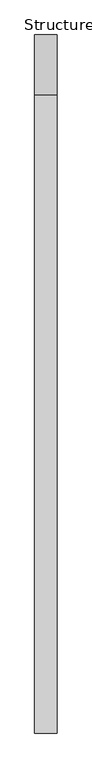
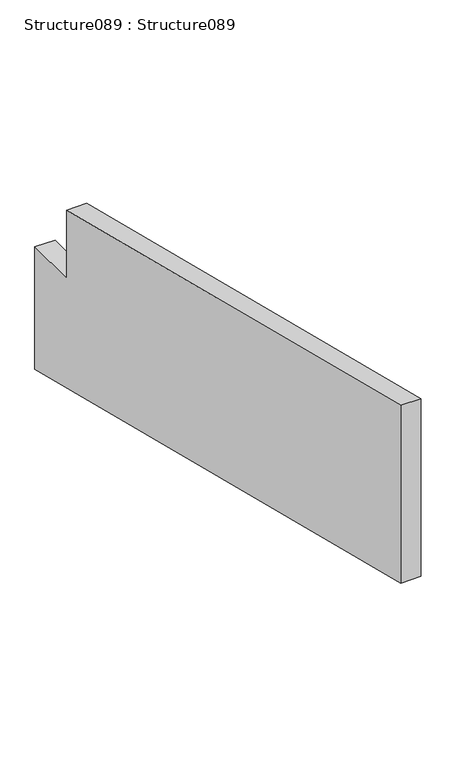
"""IFC4 building model written with IfcOpenShell, lengths in millimetres: proxy geometry, Structure089 : Structure089."""

from ifc_helpers import new_model, si_unit, frame, origin, place, context, project, spatial, polyline, outline, extrude, source, transform, mapped, element, save


def structure089_structure089_4cdf4332(model_context):
    return source(origin(), model_context, "Body", "SweptSolid", [
        extrude(outline(polyline([(3064.1094171, 41796.3564587), (4341.2980909, 41477.0623881), (4341.2980909, 41318.4021881), (4461.9480928, 41318.4021881), (4461.9480928, 41032.8236949), (3064.1094171, 41382.2833638), (3064.1094171, 41796.3564587)])), frame((1820.6861882, 0.0, 0.0), z_axis=(1.0, 0.0, 0.0), x_axis=(0.0, 1.0, 0.0)), (0.0, 0.0, 1.0), 44.45),
    ])


if __name__ == "__main__":
    model = new_model("IFC4")
    model_context = context("Model", 3, world=origin())
    ifc_project = project(units=[si_unit("LENGTHUNIT", "METRE", prefix="MILLI")], contexts=[model_context])
    site = spatial("IfcSite", under=ifc_project)
    building = spatial("IfcBuilding", under=site)
    placement = place(None, origin())
    structure089_structure089_shape = structure089_structure089_4cdf4332(model_context)
    element("IfcBuildingElementProxy", 1, Name="Structure089 : Structure089", ObjectType="Structure089 : Structure089", at=placement, inside=building, context=model_context, shape_type="MappedRepresentation", body=[
        mapped(structure089_structure089_shape, transform((0.0, 0.0, 0.0), x_axis=(1.0, 0.0, 0.0), y_axis=(0.0, 1.0, 0.0), z_axis=(0.0, 0.0, 1.0))),
    ])
    save(model, "model.ifc")

# Revit data of these elements
# Type "Structure089 : Structure089"
#   NameOverride = "Structure089"
# Element 1 (IfcBuildingElementProxy, "Structure089 : Structure089")
#   Materials on its faces: "STRUCTURAL MEMBER (SEE DWGS)"
# Materials
#   "STRUCTURAL MEMBER (SEE DWGS)": class "Unassigned", colour RGB 214 178 158, transparency 0, Cost = 0
